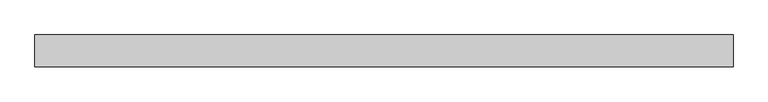
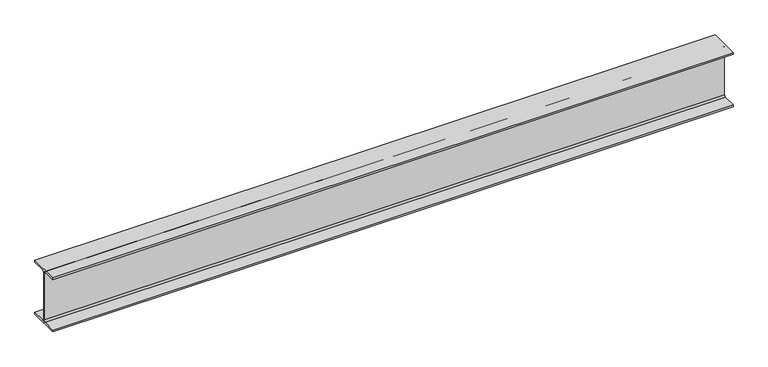
"""IFC4 building model written with IfcOpenShell, lengths in millimetres: beam geometry, Steel Beam_H-KSD3502 : H_SB_ASB_H-250x125x6x9."""

import ifcopenshell
import ifcopenshell.guid

model = None  # the IFC model being written
_history = None  # IfcOwnerHistory: only IFC2X3 demands one
_inside = {}  # id of a spatial element -> (the spatial element, [elements in it])
_under = {}  # id of a project, library or spatial element -> (it, [spatial elements below it])
_declared = {}  # id of a project -> (the project, [libraries it declares])
_typed = {}  # id of a type object -> (the type object, [elements of that type])
_made_of = {}  # id of a material, layer set ... -> (it, [elements and type objects made of it])


def new_model(schema):
    """Start an empty IFC model of exactly this schema.

    Asked for "IFC4X3", IfcOpenShell would pick the latest addendum, in which some entities
    have other attributes; the version numbers below select the first issue.
    IFC2X3 requires an IfcOwnerHistory on every rooted entity: one is made here for all.
    """
    global model, _history
    if schema == "IFC4X3":
        model = ifcopenshell.file(schema_version=(4, 3, 0, 0))
    else:
        model = ifcopenshell.file(schema=schema)
    _inside.clear()
    _under.clear()
    _declared.clear()
    _typed.clear()
    _made_of.clear()
    _history = None
    if model.schema == "IFC2X3":
        org = make("IfcOrganization", Name="unknown")
        user = make(
            "IfcPersonAndOrganization",
            ThePerson=make("IfcPerson", FamilyName="unknown"),
            TheOrganization=org,
        )
        app = make(
            "IfcApplication",
            ApplicationDeveloper=org,
            Version="unknown",
            ApplicationFullName="unknown",
            ApplicationIdentifier="unknown",
        )
        _history = make(
            "IfcOwnerHistory",
            OwningUser=user,
            OwningApplication=app,
            ChangeAction="ADDED",
            CreationDate=0,
        )
    return model


def make(cls, **values):
    """One entity of the class cls with the attributes given. An attribute that is None is left unset."""
    return model.create_entity(
        cls, **{name: value for name, value in values.items() if value is not None}
    )


def rooted(cls, **values):
    """An entity with a GlobalId (a new one), such as an element, a storey or a relation."""
    return make(cls, GlobalId=ifcopenshell.guid.new(), OwnerHistory=_history, **values)


def si_unit(unit_type, name, prefix=None):
    """IfcSIUnit, for example si_unit("LENGTHUNIT", "METRE", prefix="MILLI")."""
    return make("IfcSIUnit", UnitType=unit_type, Prefix=prefix, Name=name)


def assignment(units):
    """IfcUnitAssignment: the units of a project."""
    return None if units is None else make("IfcUnitAssignment", Units=units)


def point(xyz):
    """IfcCartesianPoint."""
    return None if xyz is None else make("IfcCartesianPoint", Coordinates=xyz)


def direction(xyz):
    """IfcDirection."""
    return None if xyz is None else make("IfcDirection", DirectionRatios=xyz)


def frame(location, z_axis=None, x_axis=None):
    """IfcAxis2Placement3D, a coordinate frame: its origin and axes. An axis left out is left unset."""
    return make(
        "IfcAxis2Placement3D",
        Location=point(location),
        Axis=direction(z_axis),
        RefDirection=direction(x_axis),
    )


def frame_2d(location, x_axis=None):
    """IfcAxis2Placement2D, a coordinate frame in the plane: its origin and x axis."""
    return make(
        "IfcAxis2Placement2D", Location=point(location), RefDirection=direction(x_axis)
    )


def origin():
    """The frame at (0, 0, 0) with its axes left unset."""
    return frame((0.0, 0.0, 0.0))


def place(relative_to, where):
    """IfcLocalPlacement: puts the frame where relative to a parent placement (None: the world)."""
    return make(
        "IfcLocalPlacement", PlacementRelTo=relative_to, RelativePlacement=where
    )


def context(
    kind, dimensions, precision=None, world=None, true_north=None, identifier=None
):
    """IfcGeometricRepresentationContext, for example the 3D "Model" context."""
    return make(
        "IfcGeometricRepresentationContext",
        ContextIdentifier=identifier,
        ContextType=kind,
        CoordinateSpaceDimension=dimensions,
        Precision=precision,
        WorldCoordinateSystem=world,
        TrueNorth=true_north,
    )


def project(units=None, contexts=None):
    """IfcProject with its units and contexts."""
    return rooted(
        "IfcProject",
        Name="project",
        RepresentationContexts=contexts,
        UnitsInContext=assignment(units),
    )


def spatial(cls, under=None, at=None, **own):
    """A site, building, storey or space (cls), placed at a placement, below another one or the project."""
    s = rooted(cls, ObjectPlacement=at, **own)
    if under is not None:
        _under.setdefault(under.id(), (under, []))[1].append(s)
    return s


def polyline(points):
    """IfcPolyline through the points."""
    return make("IfcPolyline", Points=[point(p) for p in points])


def circle_curve(where, radius):
    """IfcCircle in the frame where."""
    return make("IfcCircle", Position=where, Radius=radius)


def trimmed(basis, trim1, trim2, sense, master):
    """IfcTrimmedCurve: the piece of a basis curve between two trims."""
    return make(
        "IfcTrimmedCurve",
        BasisCurve=basis,
        Trim1=trim1,
        Trim2=trim2,
        SenseAgreement=sense,
        MasterRepresentation=master,
    )


def segment(curve, same_sense, transition):
    """IfcCompositeCurveSegment."""
    return make(
        "IfcCompositeCurveSegment",
        Transition=transition,
        SameSense=same_sense,
        ParentCurve=curve,
    )


def composite_curve(segments, self_intersect=None):
    """IfcCompositeCurve: segments joined end to end."""
    return make("IfcCompositeCurve", Segments=segments, SelfIntersect=self_intersect)


def outline(outer, holes=None, kind="AREA"):
    """IfcArbitraryClosedProfileDef: a profile drawn as a closed curve; with holes, ...WithVoids."""
    if holes is None:
        return make("IfcArbitraryClosedProfileDef", ProfileType=kind, OuterCurve=outer)
    return make(
        "IfcArbitraryProfileDefWithVoids",
        ProfileType=kind,
        OuterCurve=outer,
        InnerCurves=holes,
    )


def extrude(swept, where, along, depth):
    """IfcExtrudedAreaSolid: the profile swept, set in the frame where, extruded along a direction by depth."""
    return make(
        "IfcExtrudedAreaSolid",
        SweptArea=swept,
        Position=where,
        ExtrudedDirection=direction(along),
        Depth=depth,
    )


def shape(context_of_items, identifier, shape_type, items):
    """IfcShapeRepresentation: the items that make up one representation, for example the "Body"."""
    return make(
        "IfcShapeRepresentation",
        ContextOfItems=context_of_items,
        RepresentationIdentifier=identifier,
        RepresentationType=shape_type,
        Items=items,
    )


def source(mapping_origin, context_of_items, identifier, shape_type, items):
    """IfcRepresentationMap: a shape defined once, which mapped items show again and again."""
    return make(
        "IfcRepresentationMap",
        MappingOrigin=mapping_origin,
        MappedRepresentation=shape(context_of_items, identifier, shape_type, items),
    )


def transform(
    local_origin,
    x_axis=None,
    y_axis=None,
    z_axis=None,
    scale=None,
    scale2=None,
    scale3=None,
    uniform=True,
):
    """IfcCartesianTransformationOperator3D, or its non-uniform kind. x_axis, y_axis, z_axis: its Axis1, 2, 3."""
    if uniform:
        return make(
            "IfcCartesianTransformationOperator3D",
            Axis1=direction(x_axis),
            Axis2=direction(y_axis),
            LocalOrigin=point(local_origin),
            Scale=scale,
            Axis3=direction(z_axis),
        )
    return make(
        "IfcCartesianTransformationOperator3DnonUniform",
        Axis1=direction(x_axis),
        Axis2=direction(y_axis),
        LocalOrigin=point(local_origin),
        Scale=scale,
        Axis3=direction(z_axis),
        Scale2=scale2,
        Scale3=scale3,
    )


def mapped(mapping_source, mapping_target):
    """IfcMappedItem: shows the shape of a source again, moved by a transform."""
    return make(
        "IfcMappedItem", MappingSource=mapping_source, MappingTarget=mapping_target
    )


def made_of(thing, what):
    """Note that an element or type object is made of a material, layer set ...; save() writes the relation."""
    if what is not None:
        _made_of.setdefault(what.id(), (what, []))[1].append(thing)
    return thing


def element(
    cls,
    number,
    at=None,
    inside=None,
    cuts=None,
    type_object=None,
    material=None,
    context=None,
    identifier="Body",
    shape_type=None,
    held_by="IfcProductDefinitionShape",
    body=None,
    shapes=None,
    **own,
):
    """One element of the class cls, such as IfcWall. Its Tag is "e" and its number.

    at: its placement. inside: the storey or other place that contains it. cuts: it is an
    opening in that element (IfcRelVoidsElement). A single representation is given by context,
    identifier, shape_type and body (its items); several are given by shapes. held_by: the class
    of the entity that holds the representations. save() writes the other relations.
    """
    e = rooted(cls, Tag="e%d" % number, ObjectPlacement=at, **own)
    if body is not None:
        shapes = [shape(context, identifier, shape_type, body)]
    if shapes is not None:
        e.Representation = make(held_by, Representations=shapes)
    if inside is not None:
        _inside.setdefault(inside.id(), (inside, []))[1].append(e)
    if cuts is not None:
        rooted(
            "IfcRelVoidsElement", RelatingBuildingElement=cuts, RelatedOpeningElement=e
        )
    if type_object is not None:
        _typed.setdefault(type_object.id(), (type_object, []))[1].append(e)
    return made_of(e, material)


def aggregate(whole, parts):
    """IfcRelAggregates: a whole, such as a stair, and the parts it consists of."""
    return rooted("IfcRelAggregates", RelatingObject=whole, RelatedObjects=parts)


def save(model, path):
    """Write the relations noted so far, then the file.

    IfcRelAggregates (storeys below a building ...), IfcRelContainedInSpatialStructure (elements
    in a storey), IfcRelDefinesByType, IfcRelAssociatesMaterial and IfcRelDeclares: one each for
    every whole, place, type object, material and project.
    """
    for whole, parts in _under.values():
        aggregate(whole, parts)
    for where, things in _inside.values():
        rooted(
            "IfcRelContainedInSpatialStructure",
            RelatedElements=things,
            RelatingStructure=where,
        )
    for kind, things in _typed.values():
        rooted("IfcRelDefinesByType", RelatedObjects=things, RelatingType=kind)
    for what, things in _made_of.values():
        rooted("IfcRelAssociatesMaterial", RelatedObjects=things, RelatingMaterial=what)
    for by, libraries in _declared.values():
        rooted("IfcRelDeclares", RelatingContext=by, RelatedDefinitions=libraries)
    model.write(path)


def beam_bc66176e(model_context):
    return source(origin(), model_context, "Body", "SweptSolid", [
        extrude(outline(composite_curve([segment(polyline([(82.5, -141.5), (82.5, -151.7), (-82.5, -151.7), (-82.5, -141.5), (-11.9, -141.5)]), True, "CONTINUOUS"), segment(trimmed(circle_curve(frame_2d((-11.9, -132.6)), 8.9), [point((-11.9, -141.5))], [point((-3.0, -132.6))], True, "CARTESIAN"), True, "CONTINUOUS"), segment(polyline([(-3.0, -132.6), (-3.0, 132.6)]), True, "CONTINUOUS"), segment(trimmed(circle_curve(frame_2d((-11.9, 132.6)), 8.9), [point((-3.0, 132.6))], [point((-11.9, 141.5))], True, "CARTESIAN"), True, "CONTINUOUS"), segment(polyline([(-11.9, 141.5), (-82.5, 141.5), (-82.5, 151.7), (82.5, 151.7), (82.5, 141.5), (11.9, 141.5)]), True, "CONTINUOUS"), segment(trimmed(circle_curve(frame_2d((11.9, 132.6)), 8.9), [point((11.9, 141.5))], [point((3.0, 132.6))], True, "CARTESIAN"), True, "CONTINUOUS"), segment(polyline([(3.0, 132.6), (3.0, -132.6)]), True, "CONTINUOUS"), segment(trimmed(circle_curve(frame_2d((11.9, -132.6)), 8.9), [point((3.0, -132.6))], [point((11.9, -141.5))], True, "CARTESIAN"), True, "CONTINUOUS"), segment(polyline([(11.9, -141.5), (82.5, -141.5)]), True, "CONTINUOUS")], self_intersect=False)), frame((-1904.8, 0.0, 0.0), z_axis=(1.0, 0.0, 0.0), x_axis=(0.0, 1.0, 0.0)), (0.0, 0.0, 1.0), 3623.1833333),
    ])


if __name__ == "__main__":
    model = new_model("IFC4")
    model_context = context("Model", 3, world=origin())
    ifc_project = project(units=[si_unit("LENGTHUNIT", "METRE", prefix="MILLI")], contexts=[model_context])
    site = spatial("IfcSite", under=ifc_project)
    building = spatial("IfcBuilding", under=site)
    placement = place(None, origin())
    beam_shape = beam_bc66176e(model_context)
    element("IfcBeam", 1, ObjectType="Steel Beam_H-KSD3502 : H_SB_ASB_H-250x125x6x9", at=placement, inside=building, context=model_context, shape_type="MappedRepresentation", body=[
        mapped(beam_shape, transform((0.0, 0.0, 0.0), x_axis=(1.0, 0.0, 0.0), y_axis=(0.0, 1.0, 0.0), z_axis=(0.0, 0.0, 1.0))),
    ])
    save(model, "model.ifc")

# Revit data of these elements
# Type "Steel Beam_H-KSD3502 : H_SB_ASB_H-250x125x6x9"
#   Width = 12.5 cm
#   Web Thickness = 0.6 cm
#   Web Fillet = 1.2 cm
#   Warping Constant = 42539.8 cm⁶
#   Torsional Moment of Inertia = 7.8102 cm⁴
#   Torsional Modulus = 1.0 cm³
#   Section Area = 37.66 cm²
#   Plastic Modulus weak axis = 73.1 cm³
#   Plastic Modulus strong axis = 366.0 cm³
#   Perimeter = 0.97 m²/m
#   Nominal Weight = 29.60 kgf/m
#   Moment of Inertia weak axis = 294.00 cm⁴
#   Moment of Inertia strong axis = 4050.00 cm⁴
#   Height = 25.0 cm
#   Flange Thickness = 0.9 cm
#   Elastic Modulus weak axis = 47.0 cm³
#   Elastic Modulus strong axis = 324.0 cm³
#   Centroid Vertical = 12.5 cm
#   Centroid Horizontal = 6.25 cm
#   Length [instance default] = 1.5240 m
#   Structural Material [instance default] = Steel, 45-345
#   Assembly Code = ""
# Element 1 (IfcBeam, "Steel Beam_H-KSD3502 : H_SB_ASB_H-250x125x6x9")
#   Structural Material = none
# Materials
#   "Steel, 45-345": class "Metal", colour RGB 189 187 185, transparency 0, Description = "Steel 345 MPa", Cost = 0
